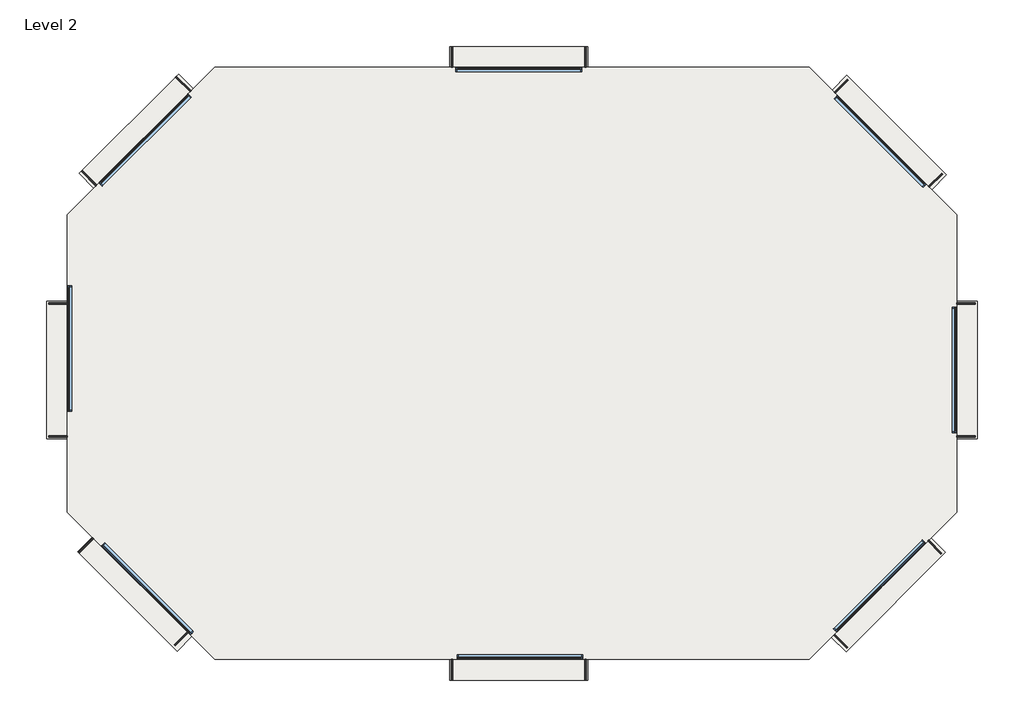
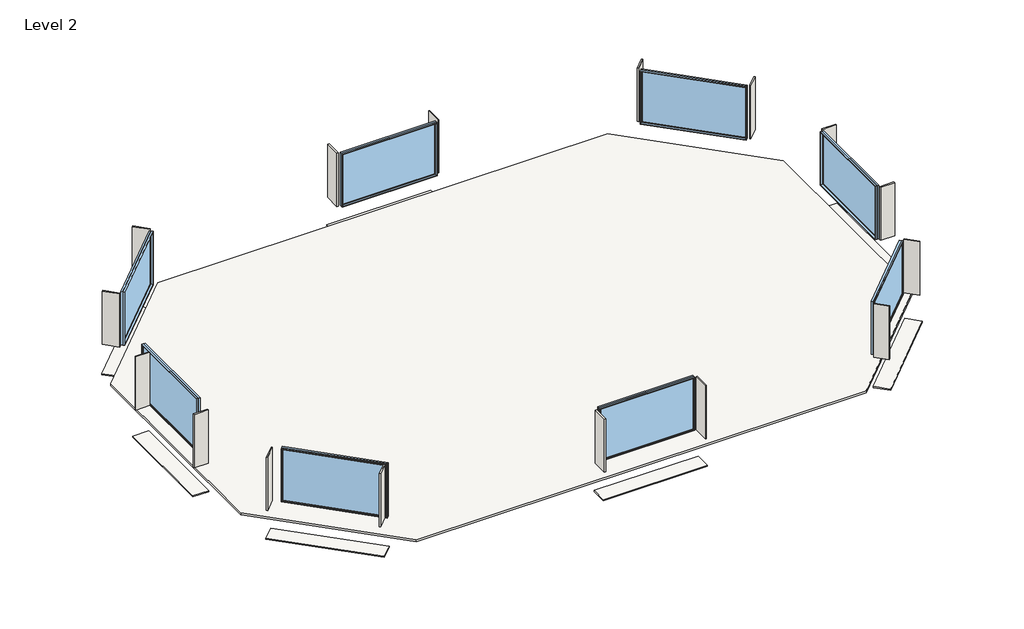
# One storey: 16 walls, 8 roofs, 8 windows, 1 slab.
"""IFC4 building model written with IfcOpenShell, lengths in millimetres."""

import ifcopenshell
import ifcopenshell.guid

model = None  # the IFC model being written
_history = None  # IfcOwnerHistory: only IFC2X3 demands one
_inside = {}  # id of a spatial element -> (the spatial element, [elements in it])
_under = {}  # id of a project, library or spatial element -> (it, [spatial elements below it])
_declared = {}  # id of a project -> (the project, [libraries it declares])
_typed = {}  # id of a type object -> (the type object, [elements of that type])
_made_of = {}  # id of a material, layer set ... -> (it, [elements and type objects made of it])


def new_model(schema):
    """Start an empty IFC model of exactly this schema.

    Asked for "IFC4X3", IfcOpenShell would pick the latest addendum, in which some entities
    have other attributes; the version numbers below select the first issue.
    IFC2X3 requires an IfcOwnerHistory on every rooted entity: one is made here for all.
    """
    global model, _history
    if schema == "IFC4X3":
        model = ifcopenshell.file(schema_version=(4, 3, 0, 0))
    else:
        model = ifcopenshell.file(schema=schema)
    _inside.clear()
    _under.clear()
    _declared.clear()
    _typed.clear()
    _made_of.clear()
    _history = None
    if model.schema == "IFC2X3":
        org = make("IfcOrganization", Name="unknown")
        user = make(
            "IfcPersonAndOrganization",
            ThePerson=make("IfcPerson", FamilyName="unknown"),
            TheOrganization=org,
        )
        app = make(
            "IfcApplication",
            ApplicationDeveloper=org,
            Version="unknown",
            ApplicationFullName="unknown",
            ApplicationIdentifier="unknown",
        )
        _history = make(
            "IfcOwnerHistory",
            OwningUser=user,
            OwningApplication=app,
            ChangeAction="ADDED",
            CreationDate=0,
        )
    return model


def make(cls, **values):
    """One entity of the class cls with the attributes given. An attribute that is None is left unset."""
    return model.create_entity(
        cls, **{name: value for name, value in values.items() if value is not None}
    )


def rooted(cls, **values):
    """An entity with a GlobalId (a new one), such as an element, a storey or a relation."""
    return make(cls, GlobalId=ifcopenshell.guid.new(), OwnerHistory=_history, **values)


def si_unit(unit_type, name, prefix=None):
    """IfcSIUnit, for example si_unit("LENGTHUNIT", "METRE", prefix="MILLI")."""
    return make("IfcSIUnit", UnitType=unit_type, Prefix=prefix, Name=name)


def assignment(units):
    """IfcUnitAssignment: the units of a project."""
    return None if units is None else make("IfcUnitAssignment", Units=units)


def point(xyz):
    """IfcCartesianPoint."""
    return None if xyz is None else make("IfcCartesianPoint", Coordinates=xyz)


def direction(xyz):
    """IfcDirection."""
    return None if xyz is None else make("IfcDirection", DirectionRatios=xyz)


def frame(location, z_axis=None, x_axis=None):
    """IfcAxis2Placement3D, a coordinate frame: its origin and axes. An axis left out is left unset."""
    return make(
        "IfcAxis2Placement3D",
        Location=point(location),
        Axis=direction(z_axis),
        RefDirection=direction(x_axis),
    )


def origin():
    """The frame at (0, 0, 0) with its axes left unset."""
    return frame((0.0, 0.0, 0.0))


def place(relative_to, where):
    """IfcLocalPlacement: puts the frame where relative to a parent placement (None: the world)."""
    return make(
        "IfcLocalPlacement", PlacementRelTo=relative_to, RelativePlacement=where
    )


def context(
    kind, dimensions, precision=None, world=None, true_north=None, identifier=None
):
    """IfcGeometricRepresentationContext, for example the 3D "Model" context."""
    return make(
        "IfcGeometricRepresentationContext",
        ContextIdentifier=identifier,
        ContextType=kind,
        CoordinateSpaceDimension=dimensions,
        Precision=precision,
        WorldCoordinateSystem=world,
        TrueNorth=true_north,
    )


def project(units=None, contexts=None):
    """IfcProject with its units and contexts."""
    return rooted(
        "IfcProject",
        Name="project",
        RepresentationContexts=contexts,
        UnitsInContext=assignment(units),
    )


def spatial(cls, under=None, at=None, **own):
    """A site, building, storey or space (cls), placed at a placement, below another one or the project."""
    s = rooted(cls, ObjectPlacement=at, **own)
    if under is not None:
        _under.setdefault(under.id(), (under, []))[1].append(s)
    return s


def polyline(points):
    """IfcPolyline through the points."""
    return make("IfcPolyline", Points=[point(p) for p in points])


def outline(outer, holes=None, kind="AREA"):
    """IfcArbitraryClosedProfileDef: a profile drawn as a closed curve; with holes, ...WithVoids."""
    if holes is None:
        return make("IfcArbitraryClosedProfileDef", ProfileType=kind, OuterCurve=outer)
    return make(
        "IfcArbitraryProfileDefWithVoids",
        ProfileType=kind,
        OuterCurve=outer,
        InnerCurves=holes,
    )


def extrude(swept, where, along, depth):
    """IfcExtrudedAreaSolid: the profile swept, set in the frame where, extruded along a direction by depth."""
    return make(
        "IfcExtrudedAreaSolid",
        SweptArea=swept,
        Position=where,
        ExtrudedDirection=direction(along),
        Depth=depth,
    )


def shape(context_of_items, identifier, shape_type, items):
    """IfcShapeRepresentation: the items that make up one representation, for example the "Body"."""
    return make(
        "IfcShapeRepresentation",
        ContextOfItems=context_of_items,
        RepresentationIdentifier=identifier,
        RepresentationType=shape_type,
        Items=items,
    )


def source(mapping_origin, context_of_items, identifier, shape_type, items):
    """IfcRepresentationMap: a shape defined once, which mapped items show again and again."""
    return make(
        "IfcRepresentationMap",
        MappingOrigin=mapping_origin,
        MappedRepresentation=shape(context_of_items, identifier, shape_type, items),
    )


def transform(
    local_origin,
    x_axis=None,
    y_axis=None,
    z_axis=None,
    scale=None,
    scale2=None,
    scale3=None,
    uniform=True,
):
    """IfcCartesianTransformationOperator3D, or its non-uniform kind. x_axis, y_axis, z_axis: its Axis1, 2, 3."""
    if uniform:
        return make(
            "IfcCartesianTransformationOperator3D",
            Axis1=direction(x_axis),
            Axis2=direction(y_axis),
            LocalOrigin=point(local_origin),
            Scale=scale,
            Axis3=direction(z_axis),
        )
    return make(
        "IfcCartesianTransformationOperator3DnonUniform",
        Axis1=direction(x_axis),
        Axis2=direction(y_axis),
        LocalOrigin=point(local_origin),
        Scale=scale,
        Axis3=direction(z_axis),
        Scale2=scale2,
        Scale3=scale3,
    )


def mapped(mapping_source, mapping_target):
    """IfcMappedItem: shows the shape of a source again, moved by a transform."""
    return make(
        "IfcMappedItem", MappingSource=mapping_source, MappingTarget=mapping_target
    )


def made_of(thing, what):
    """Note that an element or type object is made of a material, layer set ...; save() writes the relation."""
    if what is not None:
        _made_of.setdefault(what.id(), (what, []))[1].append(thing)
    return thing


def element(
    cls,
    number,
    at=None,
    inside=None,
    cuts=None,
    type_object=None,
    material=None,
    context=None,
    identifier="Body",
    shape_type=None,
    held_by="IfcProductDefinitionShape",
    body=None,
    shapes=None,
    **own,
):
    """One element of the class cls, such as IfcWall. Its Tag is "e" and its number.

    at: its placement. inside: the storey or other place that contains it. cuts: it is an
    opening in that element (IfcRelVoidsElement). A single representation is given by context,
    identifier, shape_type and body (its items); several are given by shapes. held_by: the class
    of the entity that holds the representations. save() writes the other relations.
    """
    e = rooted(cls, Tag="e%d" % number, ObjectPlacement=at, **own)
    if body is not None:
        shapes = [shape(context, identifier, shape_type, body)]
    if shapes is not None:
        e.Representation = make(held_by, Representations=shapes)
    if inside is not None:
        _inside.setdefault(inside.id(), (inside, []))[1].append(e)
    if cuts is not None:
        rooted(
            "IfcRelVoidsElement", RelatingBuildingElement=cuts, RelatedOpeningElement=e
        )
    if type_object is not None:
        _typed.setdefault(type_object.id(), (type_object, []))[1].append(e)
    return made_of(e, material)


def aggregate(whole, parts):
    """IfcRelAggregates: a whole, such as a stair, and the parts it consists of."""
    return rooted("IfcRelAggregates", RelatingObject=whole, RelatedObjects=parts)


def save(model, path):
    """Write the relations noted so far, then the file.

    IfcRelAggregates (storeys below a building ...), IfcRelContainedInSpatialStructure (elements
    in a storey), IfcRelDefinesByType, IfcRelAssociatesMaterial and IfcRelDeclares: one each for
    every whole, place, type object, material and project.
    """
    for whole, parts in _under.values():
        aggregate(whole, parts)
    for where, things in _inside.values():
        rooted(
            "IfcRelContainedInSpatialStructure",
            RelatedElements=things,
            RelatingStructure=where,
        )
    for kind, things in _typed.values():
        rooted("IfcRelDefinesByType", RelatedObjects=things, RelatingType=kind)
    for what, things in _made_of.values():
        rooted("IfcRelAssociatesMaterial", RelatedObjects=things, RelatingMaterial=what)
    for by, libraries in _declared.values():
        rooted("IfcRelDeclares", RelatingContext=by, RelatedDefinitions=libraries)
    model.write(path)


def m_fixed_2500x_4228mm_fd5e51e7(model_context):
    return source(origin(), model_context, "Body", "SweptSolid", [
        extrude(outline(polyline([(-2050.8, 54.2), (2050.8, 54.2), (2050.8, 42.2), (-2050.8, 42.2), (-2050.8, 54.2)])), frame((0.0, 0.0, 368.0), z_axis=(0.0, 0.0, 1.0), x_axis=(1.0, 0.0, 0.0)), (0.0, 0.0, 1.0), 2374.0),
        extrude(outline(polyline([(2786.0, -2094.8), (324.0, -2094.8), (324.0, 2094.8), (2786.0, 2094.8), (2786.0, -2094.8)]), holes=[polyline([(2742.0, -2050.8), (2742.0, 2050.8), (368.0, 2050.8), (368.0, -2050.8), (2742.0, -2050.8)])]), frame((0.0, 26.2, 0.0), z_axis=(0.0, 1.0, 0.0), x_axis=(0.0, 0.0, 1.0)), (0.0, 0.0, 1.0), 44.0),
        extrude(outline(polyline([(2805.0, -2113.8), (305.0, -2113.8), (305.0, 2113.8), (2805.0, 2113.8), (2805.0, -2113.8)]), holes=[polyline([(2786.0, -2094.8), (2786.0, 2094.8), (324.0, 2094.8), (324.0, -2094.8), (2786.0, -2094.8)])]), frame((0.0, 26.2, 0.0), z_axis=(0.0, 1.0, 0.0), x_axis=(0.0, 0.0, 1.0)), (0.0, 0.0, 1.0), 63.0),
        extrude(outline(polyline([(2805.0, -2113.8), (305.0, -2113.8), (305.0, 2113.8), (2805.0, 2113.8), (2805.0, -2113.8)]), holes=[polyline([(2773.0, -2081.8), (2773.0, 2081.8), (337.0, 2081.8), (337.0, -2081.8), (2773.0, -2081.8)])]), frame((0.0, -63.2, 0.0), z_axis=(0.0, 1.0, 0.0), x_axis=(0.0, 0.0, 1.0)), (0.0, 0.0, 1.0), 89.4),
    ])


model = new_model("IFC4")

# Units and contexts
model_context = context("Model", 3, world=origin())
ifc_project = project(units=[si_unit("LENGTHUNIT", "METRE", prefix="MILLI")], contexts=[model_context])

# Site, building, storey
site = spatial("IfcSite", under=ifc_project)
building = spatial("IfcBuilding", under=site)
storey = spatial("IfcBuildingStorey", under=building, Name="Level 2", Elevation=3962.4)

# Roofs
placement = place(None, origin())
element("IfcRoof", 1, ObjectType="Generic - 125mm shading", at=placement, inside=storey, context=model_context, shape_type="SweptSolid", body=[
    extrude(outline(polyline([(18552.7836697, -8602.5147149), (23180.3836697, -8602.5147149), (23180.3836697, -9302.5147149), (18552.7836697, -9302.5147149), (18552.7836697, -8602.5147149)])), frame((0.0, 0.0, 3450.0), z_axis=(0.0, 0.0, 1.0), x_axis=(1.0, 0.0, 0.0)), (0.0, 0.0, 1.0), 50.0),
])
element("IfcRoof", 2, ObjectType="Generic - 125mm shading", at=placement, inside=storey, context=model_context, shape_type="SweptSolid", body=[
    extrude(outline(polyline([(23180.3836697, 11296.9802217), (18552.7836697, 11296.9802217), (18552.7836697, 11996.9802217), (23180.3836697, 11996.9802217), (23180.3836697, 11296.9802217)])), frame((0.0, 0.0, 3450.0), z_axis=(0.0, 0.0, 1.0), x_axis=(1.0, 0.0, 0.0)), (0.0, 0.0, 1.0), 50.0),
])
element("IfcRoof", 3, ObjectType="Generic - 125mm shading", at=placement, inside=storey, context=model_context, shape_type="SweptSolid", body=[
    extrude(outline(polyline([(34745.7885808, 7190.4058824), (31403.3995039, 10532.7949592), (31895.6627273, 11025.0581826), (35238.0518042, 7682.6691057), (34745.7885808, 7190.4058824)])), frame((0.0, 0.0, 3400.0), z_axis=(0.0, 0.0, 1.0), x_axis=(1.0, 0.0, 0.0)), (0.0, 0.0, 1.0), 50.0),
])
element("IfcRoof", 4, ObjectType="Generic - 125mm shading", at=placement, inside=storey, context=model_context, shape_type="SweptSolid", body=[
    extrude(outline(polyline([(31379.6986616, -7862.0302949), (34722.0877385, -4519.641218), (35214.3509618, -5011.9044414), (31871.961885, -8354.2935183), (31379.6986616, -7862.0302949)])), frame((0.0, 0.0, 3400.0), z_axis=(0.0, 0.0, 1.0), x_axis=(1.0, 0.0, 0.0)), (0.0, 0.0, 1.0), 50.0),
])
element("IfcRoof", 5, ObjectType="Generic - 125mm shading", at=placement, inside=storey, context=model_context, shape_type="SweptSolid", body=[
    extrude(outline(polyline([(9921.2320547, 10578.9980348), (6578.8429778, 7236.6089579), (6086.5797544, 7728.8721813), (9428.9688313, 11071.2612582), (9921.2320547, 10578.9980348)])), frame((0.0, 0.0, 3400.0), z_axis=(0.0, 0.0, 1.0), x_axis=(1.0, 0.0, 0.0)), (0.0, 0.0, 1.0), 50.0),
])
element("IfcRoof", 6, ObjectType="Generic - 125mm shading", at=placement, inside=storey, context=model_context, shape_type="SweptSolid", body=[
    extrude(outline(polyline([(6532.6399022, -4495.9403757), (9875.0289791, -7838.3294525), (9382.7657557, -8330.5926759), (6040.3766789, -4988.203599), (6532.6399022, -4495.9403757)])), frame((0.0, 0.0, 3400.0), z_axis=(0.0, 0.0, 1.0), x_axis=(1.0, 0.0, 0.0)), (0.0, 0.0, 1.0), 50.0),
])
element("IfcRoof", 7, ObjectType="Generic - 125mm shading", at=placement, inside=storey, context=model_context, shape_type="SweptSolid", body=[
    extrude(outline(polyline([(35588.9617098, -1191.3598794), (35588.9617098, 3436.2401206), (36288.9617098, 3436.2401206), (36288.9617098, -1191.3598794), (35588.9617098, -1191.3598794)])), frame((0.0, 0.0, 3450.0), z_axis=(0.0, 0.0, 1.0), x_axis=(1.0, 0.0, 0.0)), (0.0, 0.0, 1.0), 50.0),
])
element("IfcRoof", 8, ObjectType="Generic - 125mm shading", at=placement, inside=storey, context=model_context, shape_type="SweptSolid", body=[
    extrude(outline(polyline([(5689.4667732, 3436.2401206), (5689.4667732, -1191.3598794), (4989.4667732, -1191.3598794), (4989.4667732, 3436.2401206), (5689.4667732, 3436.2401206)])), frame((0.0, 0.0, 3450.0), z_axis=(0.0, 0.0, 1.0), x_axis=(1.0, 0.0, 0.0)), (0.0, 0.0, 1.0), 50.0),
])

# Slab
element("IfcSlab", 9, ObjectType="Generic Floor - 100mm", at=placement, inside=storey, context=model_context, shape_type="SweptSolid", body=[
    extrude(outline(polyline([(10639.2142415, 11296.9802217), (30639.2142415, 11296.9802217), (35588.9617098, 6347.2327534), (35588.9617098, -3652.7672466), (30639.2142415, -8602.5147149), (10639.2142415, -8602.5147149), (5689.4667732, -3652.7672466), (5689.4667732, 6347.2327534), (10639.2142415, 11296.9802217)])), frame((0.0, 0.0, 3862.4), z_axis=(0.0, 0.0, 1.0), x_axis=(1.0, 0.0, 0.0)), (0.0, 0.0, 1.0), 100.0),
])

# Walls
element("IfcWall", 10, ObjectType="Generic - Shading", at=placement, inside=storey, context=model_context, shape_type="SweptSolid", body=[
    extrude(outline(polyline([(18602.7836697, -9302.5147149), (18602.7836697, -8602.5147149), (18652.7836697, -8602.5147149), (18652.7836697, -9302.5147149), (18602.7836697, -9302.5147149)])), frame((0.0, 0.0, 4762.4), z_axis=(0.0, 0.0, 1.0), x_axis=(1.0, 0.0, 0.0)), (0.0, 0.0, 1.0), 2500.0),
])
element("IfcWall", 11, ObjectType="Generic - Shading", at=placement, inside=storey, context=model_context, shape_type="SweptSolid", body=[
    extrude(outline(polyline([(23080.3836697, -9302.5147149), (23080.3836697, -8602.5147149), (23130.3836697, -8602.5147149), (23130.3836697, -9302.5147149), (23080.3836697, -9302.5147149)])), frame((0.0, 0.0, 4762.4), z_axis=(0.0, 0.0, 1.0), x_axis=(1.0, 0.0, 0.0)), (0.0, 0.0, 1.0), 2500.0),
])
element("IfcWall", 12, ObjectType="Generic - Shading", at=placement, inside=storey, context=model_context, shape_type="SweptSolid", body=[
    extrude(outline(polyline([(18652.7836697, 11996.9802217), (18652.7836697, 11296.9802217), (18602.7836697, 11296.9802217), (18602.7836697, 11996.9802217), (18652.7836697, 11996.9802217)])), frame((0.0, 0.0, 4762.4), z_axis=(0.0, 0.0, 1.0), x_axis=(1.0, 0.0, 0.0)), (0.0, 0.0, 1.0), 2500.0),
])
element("IfcWall", 13, ObjectType="Generic - Shading", at=placement, inside=storey, context=model_context, shape_type="SweptSolid", body=[
    extrude(outline(polyline([(23130.3836697, 11996.9802217), (23130.3836697, 11296.9802217), (23080.3836697, 11296.9802217), (23080.3836697, 11996.9802217), (23130.3836697, 11996.9802217)])), frame((0.0, 0.0, 4762.4), z_axis=(0.0, 0.0, 1.0), x_axis=(1.0, 0.0, 0.0)), (0.0, 0.0, 1.0), 2500.0),
])
element("IfcWall", 14, ObjectType="Generic - Shading", at=placement, inside=storey, context=model_context, shape_type="SweptSolid", body=[
    extrude(outline(polyline([(31949.4844771, 10868.8964063), (31508.391267, 10427.8031962), (31473.035928, 10463.1585352), (31914.1291381, 10904.2517453), (31949.4844771, 10868.8964063)])), frame((0.0, 0.0, 4762.4), z_axis=(0.0, 0.0, 1.0), x_axis=(1.0, 0.0, 0.0)), (0.0, 0.0, 1.0), 2500.0),
])
element("IfcWall", 15, ObjectType="Generic - Shading", at=placement, inside=storey, context=model_context, shape_type="SweptSolid", body=[
    extrude(outline(polyline([(35116.1711128, 7702.2097706), (34675.0779027, 7261.1165605), (34639.7225636, 7296.4718995), (35080.8157737, 7737.5651097), (35116.1711128, 7702.2097706)])), frame((0.0, 0.0, 4762.4), z_axis=(0.0, 0.0, 1.0), x_axis=(1.0, 0.0, 0.0)), (0.0, 0.0, 1.0), 2500.0),
])
element("IfcWall", 16, ObjectType="Generic - Shading", at=placement, inside=storey, context=model_context, shape_type="SweptSolid", body=[
    extrude(outline(polyline([(31890.4282957, -8233.487081), (31449.3350856, -7792.3938709), (31484.6904247, -7757.0385318), (31925.7836348, -8198.1317419), (31890.4282957, -8233.487081)])), frame((0.0, 0.0, 4762.4), z_axis=(0.0, 0.0, 1.0), x_axis=(1.0, 0.0, 0.0)), (0.0, 0.0, 1.0), 2500.0),
])
element("IfcWall", 17, ObjectType="Generic - Shading", at=placement, inside=storey, context=model_context, shape_type="SweptSolid", body=[
    extrude(outline(polyline([(35057.1149314, -5066.8004453), (34616.0217213, -4625.7072352), (34651.3770603, -4590.3518961), (35092.4702705, -5031.4451062), (35057.1149314, -5066.8004453)])), frame((0.0, 0.0, 4762.4), z_axis=(0.0, 0.0, 1.0), x_axis=(1.0, 0.0, 0.0)), (0.0, 0.0, 1.0), 2500.0),
])
element("IfcWall", 18, ObjectType="Generic - Shading", at=placement, inside=storey, context=model_context, shape_type="SweptSolid", body=[
    extrude(outline(polyline([(9356.6208838, 11004.3363576), (9851.5956306, 10509.3616108), (9816.2402916, 10474.0062717), (9321.2655447, 10968.9810185), (9356.6208838, 11004.3363576)])), frame((0.0, 0.0, 4762.4), z_axis=(0.0, 0.0, 1.0), x_axis=(1.0, 0.0, 0.0)), (0.0, 0.0, 1.0), 2500.0),
])
element("IfcWall", 19, ObjectType="Generic - Shading", at=placement, inside=storey, context=model_context, shape_type="SweptSolid", body=[
    extrude(outline(polyline([(6189.9342481, 7837.6497219), (6684.908995, 7342.6749751), (6649.5536559, 7307.319636), (6154.5789091, 7802.2943829), (6189.9342481, 7837.6497219)])), frame((0.0, 0.0, 4762.4), z_axis=(0.0, 0.0, 1.0), x_axis=(1.0, 0.0, 0.0)), (0.0, 0.0, 1.0), 2500.0),
])
element("IfcWall", 20, ObjectType="Generic - Shading", at=placement, inside=storey, context=model_context, shape_type="SweptSolid", body=[
    extrude(outline(polyline([(9275.0624692, -8120.5493628), (9716.1556793, -7679.4561527), (9751.5110184, -7714.8114918), (9310.4178082, -8155.9047019), (9275.0624692, -8120.5493628)])), frame((0.0, 0.0, 4762.4), z_axis=(0.0, 0.0, 1.0), x_axis=(1.0, 0.0, 0.0)), (0.0, 0.0, 1.0), 2500.0),
])
element("IfcWall", 21, ObjectType="Generic - Shading", at=placement, inside=storey, context=model_context, shape_type="SweptSolid", body=[
    extrude(outline(polyline([(6054.4942968, -5007.7442639), (6549.4690436, -4512.769517), (6584.8243827, -4548.1248561), (6089.8496359, -5043.0996029), (6054.4942968, -5007.7442639)])), frame((0.0, 0.0, 4762.4), z_axis=(0.0, 0.0, 1.0), x_axis=(1.0, 0.0, 0.0)), (0.0, 0.0, 1.0), 2500.0),
])
element("IfcWall", 22, ObjectType="Generic - Shading", at=placement, inside=storey, context=model_context, shape_type="SweptSolid", body=[
    extrude(outline(polyline([(36212.7617098, -1141.3598794), (35588.9617098, -1141.3598794), (35588.9617098, -1091.3598794), (36212.7617098, -1091.3598794), (36212.7617098, -1141.3598794)])), frame((0.0, 0.0, 4762.4), z_axis=(0.0, 0.0, 1.0), x_axis=(1.0, 0.0, 0.0)), (0.0, 0.0, 1.0), 2500.0),
])
element("IfcWall", 23, ObjectType="Generic - Shading", at=placement, inside=storey, context=model_context, shape_type="SweptSolid", body=[
    extrude(outline(polyline([(36212.7617098, 3336.2401206), (35588.9617098, 3336.2401206), (35588.9617098, 3386.2401206), (36212.7617098, 3386.2401206), (36212.7617098, 3336.2401206)])), frame((0.0, 0.0, 4762.4), z_axis=(0.0, 0.0, 1.0), x_axis=(1.0, 0.0, 0.0)), (0.0, 0.0, 1.0), 2500.0),
])
element("IfcWall", 24, ObjectType="Generic - Shading", at=placement, inside=storey, context=model_context, shape_type="SweptSolid", body=[
    extrude(outline(polyline([(5065.6667732, -1091.3598794), (5689.4667732, -1091.3598794), (5689.4667732, -1141.3598794), (5065.6667732, -1141.3598794), (5065.6667732, -1091.3598794)])), frame((0.0, 0.0, 4762.4), z_axis=(0.0, 0.0, 1.0), x_axis=(1.0, 0.0, 0.0)), (0.0, 0.0, 1.0), 2500.0),
])
element("IfcWall", 25, ObjectType="Generic - Shading", at=placement, inside=storey, context=model_context, shape_type="SweptSolid", body=[
    extrude(outline(polyline([(5065.6667732, 3386.2401206), (5689.4667732, 3386.2401206), (5689.4667732, 3336.2401206), (5065.6667732, 3336.2401206), (5065.6667732, 3386.2401206)])), frame((0.0, 0.0, 4762.4), z_axis=(0.0, 0.0, 1.0), x_axis=(1.0, 0.0, 0.0)), (0.0, 0.0, 1.0), 2500.0),
])

# Windows
m_fixed_2500x_4228mm_shape = m_fixed_2500x_4228mm_fd5e51e7(model_context)
element("IfcWindow", 26, ObjectType="M_Fixed : 2500X 4228mm", at=placement, inside=storey, context=model_context, shape_type="MappedRepresentation", body=[
    mapped(m_fixed_2500x_4228mm_shape, transform((20907.1791073, -8513.3147149, 4457.4), x_axis=(-1.0, 0.0, 0.0), y_axis=(0.0, -1.0, 0.0), z_axis=(0.0, 0.0, 1.0))),
])
element("IfcWindow", 27, ObjectType="M_Fixed : 2500X 4228mm", at=placement, inside=storey, context=model_context, shape_type="MappedRepresentation", body=[
    mapped(m_fixed_2500x_4228mm_shape, transform((32987.5548042, -6128.0263025, 4457.4), x_axis=(-0.707106781186548, -0.7071067811865471, 0.0), y_axis=(0.7071067811865471, -0.707106781186548, 0.0), z_axis=(0.0, 0.0, 1.0))),
])
element("IfcWindow", 28, ObjectType="M_Fixed : 2500X 4228mm", at=placement, inside=storey, context=model_context, shape_type="MappedRepresentation", body=[
    mapped(m_fixed_2500x_4228mm_shape, transform((35499.7617098, 1122.4401206, 4457.4), x_axis=(0.0, -1.0, 0.0), y_axis=(1.0, 0.0, 0.0), z_axis=(0.0, 0.0, 1.0))),
])
element("IfcWindow", 29, ObjectType="M_Fixed : 2500X 4228mm", at=placement, inside=storey, context=model_context, shape_type="MappedRepresentation", body=[
    mapped(m_fixed_2500x_4228mm_shape, transform((33011.2556466, 8798.7909669, 4457.4), x_axis=(0.7071067811865468, -0.7071067811865483, 0.0), y_axis=(0.7071067811865483, 0.7071067811865468, 0.0), z_axis=(0.0, 0.0, 1.0))),
])
element("IfcWindow", 30, ObjectType="M_Fixed : 2500X 4228mm", at=placement, inside=storey, context=model_context, shape_type="MappedRepresentation", body=[
    mapped(m_fixed_2500x_4228mm_shape, transform((20866.5836697, 11207.7802217, 4457.4), x_axis=(1.0, 0.0, 0.0), y_axis=(0.0, 1.0, 0.0), z_axis=(0.0, 0.0, 1.0))),
])
element("IfcWindow", 31, ObjectType="M_Fixed : 2500X 4228mm", at=placement, inside=storey, context=model_context, shape_type="MappedRepresentation", body=[
    mapped(m_fixed_2500x_4228mm_shape, transform((8313.375912, 8844.9940424, 4457.4), x_axis=(0.7071067811865479, 0.707106781186547, 0.0), y_axis=(-0.707106781186547, 0.7071067811865479, 0.0), z_axis=(0.0, 0.0, 1.0))),
])
element("IfcWindow", 32, ObjectType="M_Fixed : 2500X 4228mm", at=placement, inside=storey, context=model_context, shape_type="MappedRepresentation", body=[
    mapped(m_fixed_2500x_4228mm_shape, transform((5778.6667732, 1842.808734, 4457.4), x_axis=(0.0, 1.0, 0.0), y_axis=(-1.0, 0.0, 0.0), z_axis=(0.0, 0.0, 1.0))),
])
element("IfcWindow", 33, ObjectType="M_Fixed : 2500X 4228mm", at=placement, inside=storey, context=model_context, shape_type="MappedRepresentation", body=[
    mapped(m_fixed_2500x_4228mm_shape, transform((8388.5493935, -6225.7020172, 4457.4), x_axis=(-0.707106781186546, 0.707106781186549, 0.0), y_axis=(-0.707106781186549, -0.707106781186546, 0.0), z_axis=(0.0, 0.0, 1.0))),
])

save(model, "model.ifc")

# Revit data of these elements
# Type "Generic - 125mm shading"
#   Layers, outside or top first: 50 mm no material (function 1)
# Type "Generic Floor - 100mm"
#   Function = 0
#   Layers, outside or top first: 100 mm no material (function 1)
# Type "Generic - Shading"
#   Layers, outside or top first: 50 mm no material (function 1)
# Type "M_Fixed : 2500X 4228mm"
#   Type Mark = "25"
#   Height = 2500 mm
#   Default Sill Height = 305 mm
#   Width = 4227.6 mm
#   Window Inset = 19 mm
#   Frame Exterior Material = Sash
#   Frame Interior Material = Sash
#   Glass Pane Material = Glass
#   Sash = Sash
#   Wall Closure = (empty or 0)
# Elements 1, 2, 7, 8 (IfcRoof, "Generic - 125mm shading")
#   built-in parameter 1001705 = 11.4829 (stored number, unit not read)
#   built-in parameter 1001701 = -1.6811 (stored number, unit not read)
#   built-in parameter 1001710 = 33615
#   Phase Created = New Construction
#   Materials on its faces: "Default Roof"
# Elements 3, 4, 5, 6 (IfcRoof, "Generic - 125mm shading")
#   built-in parameter 1001705 = 11.3189 (stored number, unit not read)
#   built-in parameter 1001701 = -1.84514 (stored number, unit not read)
#   built-in parameter 1001710 = 33615
#   Phase Created = New Construction
#   Materials on its faces: "Default Roof"
# Element 9 (IfcSlab, "Generic Floor - 100mm")
#   built-in parameter 1001955 = 0.785398 (stored number, unit not read)
#   Height Offset From Level = 0 mm
#   Phase Created = New Construction
#   Materials on its faces: "Default Floor"
# Elements 10, 11, 12, 13, 14, 15, 16, 17, 18, 19, 20, 21, 22, 23, 24, 25 (IfcWall, "Generic - Shading")
#   built-in parameter 1001111 = 800 mm
#   Top Offset = -662.4 mm
#   Base Offset = 800 mm
#   wall height = 2500 mm
#   Phase Created = New Construction
#   Base Constraint = Level 2
#   Top Constraint = Roof Level
#   Materials on its faces: "Default Wall"
# Element 26 (IfcWindow, "M_Fixed : 2500X 4228mm")
#   Mark = "23"
#   Phase Created = New Construction
#   Materials on its faces: "Sash", "Glass"
# Element 27 (IfcWindow, "M_Fixed : 2500X 4228mm")
#   Mark = "24"
#   Phase Created = New Construction
#   Materials on its faces: "Sash", "Glass"
# Element 28 (IfcWindow, "M_Fixed : 2500X 4228mm")
#   Mark = "26"
#   Phase Created = New Construction
#   Materials on its faces: "Sash", "Glass"
# Element 29 (IfcWindow, "M_Fixed : 2500X 4228mm")
#   Mark = "33"
#   Phase Created = New Construction
#   Materials on its faces: "Sash", "Glass"
# Element 30 (IfcWindow, "M_Fixed : 2500X 4228mm")
#   Mark = "34"
#   Phase Created = New Construction
#   Materials on its faces: "Sash", "Glass"
# Element 31 (IfcWindow, "M_Fixed : 2500X 4228mm")
#   Mark = "35"
#   Phase Created = New Construction
#   Materials on its faces: "Sash", "Glass"
# Element 32 (IfcWindow, "M_Fixed : 2500X 4228mm")
#   Mark = "36"
#   Phase Created = New Construction
#   Materials on its faces: "Sash", "Glass"
# Element 33 (IfcWindow, "M_Fixed : 2500X 4228mm")
#   Mark = "37"
#   Phase Created = New Construction
#   Materials on its faces: "Sash", "Glass"
# Materials
#   "Sash": class "Wood", colour RGB 136 99 55, transparency 0
#   "Glass": class "Glass", colour RGB 0 128 192, transparency 0.9, Description = "Soda Lime Glass", Cost = 0
#   "Default Roof": class "Miscellaneous", colour RGB 0 127 0, transparency 0, Cost = 0
#   "Default Floor": class "Miscellaneous", colour RGB 127 127 127, transparency 0, Cost = 0
#   "Default Wall": class "Miscellaneous", colour RGB 128 128 128, transparency 0, Cost = 0
# Room at (21789.452, 2355.414) mm, phase "New Construction", upper level "Level 2", upper offset 3962.4 mm, lower offset 0 mm
#   Number = "12"
#   Name = "Room"
